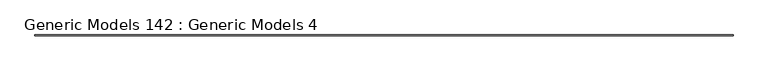
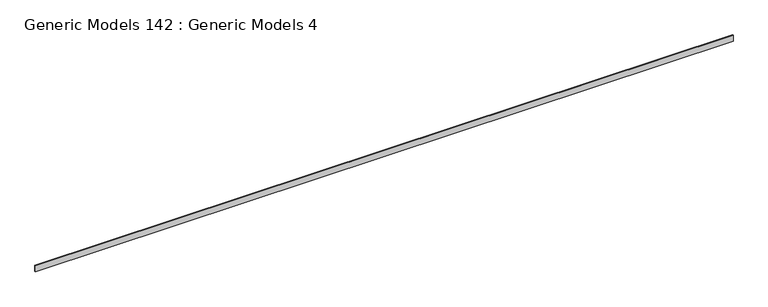
"""IFC4 building model written with IfcOpenShell, lengths in millimetres: proxy geometry, Generic Models 142 : Generic Models 4."""

from ifc_helpers import new_model, si_unit, frame, origin, place, context, project, spatial, polyline, outline, extrude, source, transform, mapped, element, save


def generic_models_142_generic_models_4_bf06cd15(model_context):
    return source(origin(), model_context, "Body", "SweptSolid", [
        extrude(outline(polyline([(20644.6159513, 7056.3254549), (20644.6159513, 7069.0254549), (33192.2159513, 7069.0254549), (33192.2159513, 7056.3254549), (20644.6159513, 7056.3254549)])), frame((0.0, 0.0, 123786.1261094), z_axis=(0.0, 0.0, 1.0), x_axis=(1.0, 0.0, 0.0)), (0.0, 0.0, 1.0), 114.3112934),
    ])


if __name__ == "__main__":
    model = new_model("IFC4")
    model_context = context("Model", 3, world=origin())
    ifc_project = project(units=[si_unit("LENGTHUNIT", "METRE", prefix="MILLI")], contexts=[model_context])
    site = spatial("IfcSite", under=ifc_project)
    building = spatial("IfcBuilding", under=site)
    placement = place(None, origin())
    generic_models_142_generic_models_4_shape = generic_models_142_generic_models_4_bf06cd15(model_context)
    element("IfcBuildingElementProxy", 1, Name="Generic Models 142 : Generic Models 4", ObjectType="Generic Models 142 : Generic Models 4", at=placement, inside=building, context=model_context, shape_type="MappedRepresentation", body=[
        mapped(generic_models_142_generic_models_4_shape, transform((0.0, 0.0, 0.0), x_axis=(1.0, 0.0, 0.0), y_axis=(0.0, 1.0, 0.0), z_axis=(0.0, 0.0, 1.0))),
    ])
    save(model, "model.ifc")

# Revit data of these elements
# Element 1 (IfcBuildingElementProxy, "Generic Models 142 : Generic Models 4")
#   Materials on its faces: "_CONCRETE EXPANSION JOINT - MINERAL FIBER"
# Materials
#   "_CONCRETE EXPANSION JOINT - MINERAL FIBER": class "Generic", colour RGB 190 220 196, transparency 0, Cost = 0
